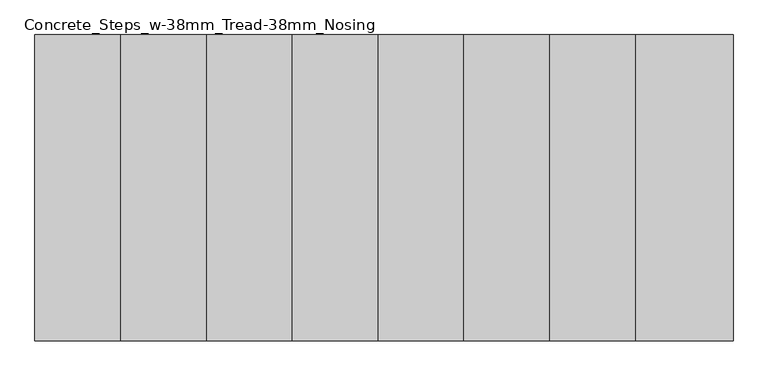
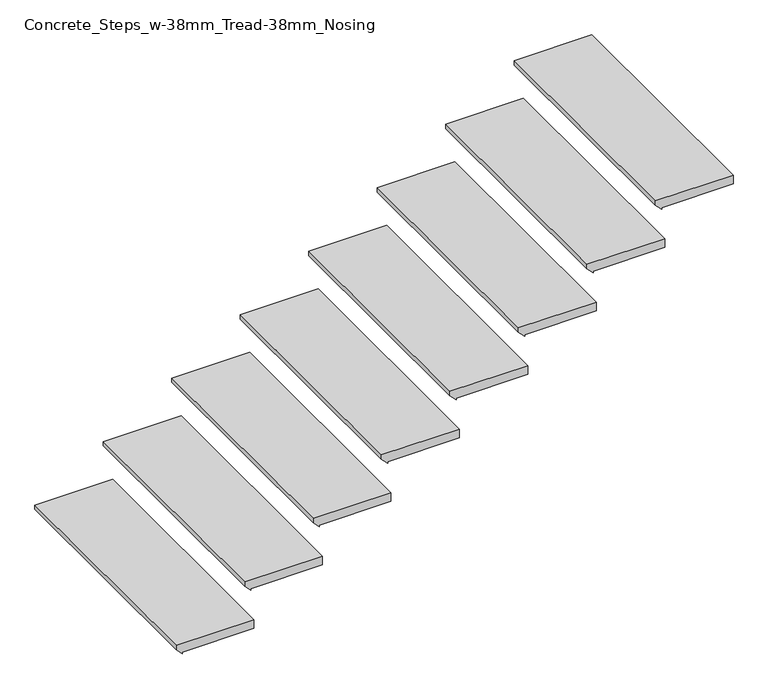
"""IFC4 building model written with IfcOpenShell, lengths in millimetres: stair flight geometry, Concrete_Steps_w-38mm_Tread-38mm_Nosing."""

from ifc_helpers import new_model, si_unit, frame, origin, place, context, project, spatial, polyline, outline, extrude, source, transform, mapped, element, save


def concrete_steps_w_38mm_tread_38mm_nosing_ba25514f(model_context):
    return source(origin(), model_context, "Body", "SweptSolid", [
        extrude(outline(polyline([(1588.2352941, -2616.2155657), (1588.2352941, -2934.2155657), (1569.1852941, -2934.2155657), (1543.7852941, -2908.8155657), (1550.2352941, -2908.8155657), (1550.2352941, -2616.2155657), (1588.2352941, -2616.2155657)])), frame((0.0, 8211.7063821, 0.0), z_axis=(0.0, 1.0, 0.0), x_axis=(0.0, 0.0, 1.0)), (0.0, 0.0, 1.0), 1000.0),
        extrude(outline(polyline([(1764.7058824, -2336.2155657), (1764.7058824, -2654.2155657), (1745.6558824, -2654.2155657), (1720.2558824, -2628.8155657), (1726.7058824, -2628.8155657), (1726.7058824, -2336.2155657), (1764.7058824, -2336.2155657)])), frame((0.0, 8211.7063821, 0.0), z_axis=(0.0, 1.0, 0.0), x_axis=(0.0, 0.0, 1.0)), (0.0, 0.0, 1.0), 1000.0),
        extrude(outline(polyline([(1941.1764706, -2056.2155657), (1941.1764706, -2374.2155657), (1922.1264706, -2374.2155657), (1896.7264706, -2348.8155657), (1903.1764706, -2348.8155657), (1903.1764706, -2056.2155657), (1941.1764706, -2056.2155657)])), frame((0.0, 8211.7063821, 0.0), z_axis=(0.0, 1.0, 0.0), x_axis=(0.0, 0.0, 1.0)), (0.0, 0.0, 1.0), 1000.0),
        extrude(outline(polyline([(2117.6470588, -1776.2155657), (2117.6470588, -2094.2155657), (2098.5970588, -2094.2155657), (2073.1970588, -2068.8155657), (2079.6470588, -2068.8155657), (2079.6470588, -1776.2155657), (2117.6470588, -1776.2155657)])), frame((0.0, 8211.7063821, 0.0), z_axis=(0.0, 1.0, 0.0), x_axis=(0.0, 0.0, 1.0)), (0.0, 0.0, 1.0), 1000.0),
        extrude(outline(polyline([(2294.1176471, -1496.2155657), (2294.1176471, -1814.2155657), (2275.0676471, -1814.2155657), (2249.6676471, -1788.8155657), (2256.1176471, -1788.8155657), (2256.1176471, -1496.2155657), (2294.1176471, -1496.2155657)])), frame((0.0, 8211.7063821, 0.0), z_axis=(0.0, 1.0, 0.0), x_axis=(0.0, 0.0, 1.0)), (0.0, 0.0, 1.0), 1000.0),
        extrude(outline(polyline([(2470.5882353, -1216.2155657), (2470.5882353, -1534.2155657), (2451.5382353, -1534.2155657), (2426.1382353, -1508.8155657), (2432.5882353, -1508.8155657), (2432.5882353, -1216.2155657), (2470.5882353, -1216.2155657)])), frame((0.0, 8211.7063821, 0.0), z_axis=(0.0, 1.0, 0.0), x_axis=(0.0, 0.0, 1.0)), (0.0, 0.0, 1.0), 1000.0),
        extrude(outline(polyline([(2647.0588235, -936.2155657), (2647.0588235, -1254.2155657), (2628.0088235, -1254.2155657), (2602.6088235, -1228.8155657), (2609.0588235, -1228.8155657), (2609.0588235, -936.2155657), (2647.0588235, -936.2155657)])), frame((0.0, 8211.7063821, 0.0), z_axis=(0.0, 1.0, 0.0), x_axis=(0.0, 0.0, 1.0)), (0.0, 0.0, 1.0), 1000.0),
        extrude(outline(polyline([(2823.5294118, -656.2155657), (2823.5294118, -974.2155657), (2804.4794118, -974.2155657), (2779.0794118, -948.8155657), (2785.5294118, -948.8155657), (2785.5294118, -656.2155657), (2823.5294118, -656.2155657)])), frame((0.0, 8211.7063821, 0.0), z_axis=(0.0, 1.0, 0.0), x_axis=(0.0, 0.0, 1.0)), (0.0, 0.0, 1.0), 1000.0),
    ])


if __name__ == "__main__":
    model = new_model("IFC4")
    model_context = context("Model", 3, world=origin())
    ifc_project = project(units=[si_unit("LENGTHUNIT", "METRE", prefix="MILLI")], contexts=[model_context])
    site = spatial("IfcSite", under=ifc_project)
    building = spatial("IfcBuilding", under=site)
    placement = place(None, origin())
    concrete_steps_w_38mm_tread_38mm_nosing_shape = concrete_steps_w_38mm_tread_38mm_nosing_ba25514f(model_context)
    element("IfcStairFlight", 1, ObjectType="Concrete_Steps_w-38mm_Tread-38mm_Nosing", at=placement, inside=building, context=model_context, shape_type="MappedRepresentation", body=[
        mapped(concrete_steps_w_38mm_tread_38mm_nosing_shape, transform((0.0, 0.0, 0.0), x_axis=(1.0, 0.0, 0.0), y_axis=(0.0, 1.0, 0.0), z_axis=(0.0, 0.0, 1.0))),
    ])
    save(model, "model.ifc")

# Revit data of these elements
# Element 1 (IfcStairFlight, "Concrete_Steps_w-38mm_Tread-38mm_Nosing")
#   Materials on its faces: "Concrete, Cast-in-Place gray"
# Materials
#   "Concrete, Cast-in-Place gray": class "Concrete", colour RGB 192 192 192, transparency 0, Description = "Cast-in-place concrete", Cost = 0
